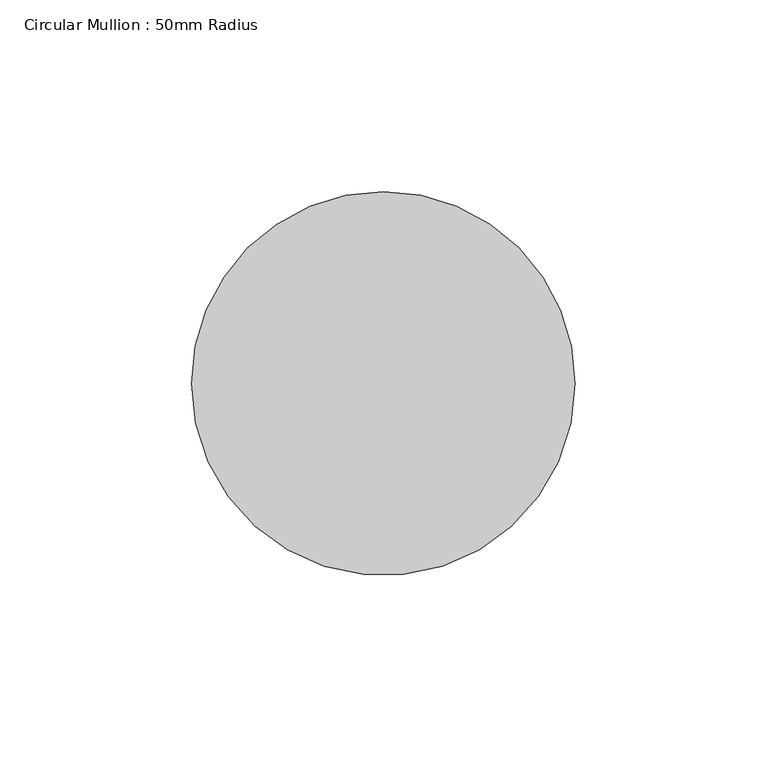
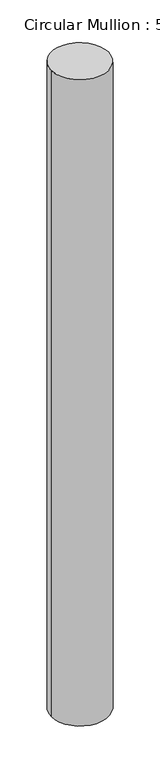
"""IFC4 building model written with IfcOpenShell, lengths in millimetres: member geometry, Circular Mullion : 50mm Radius."""

from ifc_helpers import new_model, si_unit, frame, origin, place, context, project, spatial, ellipse_curve, source, transform, mapped, element, save
from ifc_brep_helpers import plane_surface, cylinder_surface, advanced_brep


def circular_mullion_50mm_radius_43a44cb1(model_context):
    return source(origin(), model_context, "Body", "AdvancedBrep", [
        advanced_brep(
        [(-100.0, 0.0, 0.8091745), (0.0, 0.0, 0.0), (0.0, 0.0, -1191.2930542), (-100.0, 0.0, -1192.1357191)],
        [
            (0, 1, ellipse_curve(frame((-50.0, 0.0, 0.4045872), z_axis=(-0.00809072290162807, -0.013678510149129876, -0.9998737113070977), x_axis=(-0.5090365390349583, -0.8605981875941529, 0.015892181630306954)), 50.0063152, 50.0)),
            (1, 2),
            (2, 3, ellipse_curve(frame((-50.0, 0.0, -1191.7143867), z_axis=(-0.008425494316828716, -0.014244488524133757, 0.9998630434175488), x_axis=(0.5090311080034745, 0.8605890056681867, 0.016549755520753683)), 50.0068488, 50.0)),
            (3, 0),
            (1, 0, ellipse_curve(frame((-50.0, 0.0, 0.4045872), z_axis=(-0.00809072290162807, -0.013678510149129876, -0.9998737113070977), x_axis=(-0.5090365390349583, -0.8605981875941529, 0.015892181630306954)), 50.0063152, 50.0)),
            (3, 2, ellipse_curve(frame((-50.0, 0.0, -1191.7143867), z_axis=(-0.008425494316828716, -0.014244488524133757, 0.9998630434175488), x_axis=(0.5090311080034745, 0.8605890056681867, 0.016549755520753683)), 50.0068488, 50.0)),
        ],
        [
            cylinder_surface(frame((-50.0, 0.0, 0.0), z_axis=(0.0, 0.0, 1.0), x_axis=(1.0, 0.0, 0.0)), 50.0),
            plane_surface(frame((-262.3434586, 155.1739338, 0.0), z_axis=(0.00809072290162807, 0.013678510149129876, 0.9998737113070977), x_axis=(0.5090365390349586, 0.8605981875941526, -0.015892181630310483))),
            plane_surface(frame((-262.3434586, 155.1739338, -1191.2930542), z_axis=(0.008425494316828716, 0.014244488524133757, -0.9998630434175488), x_axis=(0.5090311080034744, 0.8605890056681866, 0.01654975552076499))),
        ],
        [
            (0, [[1, 2, 3, 4]]),
            (0, [[5, -4, 6, -2]]),
            (1, [[-1, -5]]),
            (2, [[-6, -3]]),
        ],
    ),
    ])


if __name__ == "__main__":
    model = new_model("IFC4")
    model_context = context("Model", 3, world=origin())
    ifc_project = project(units=[si_unit("LENGTHUNIT", "METRE", prefix="MILLI")], contexts=[model_context])
    site = spatial("IfcSite", under=ifc_project)
    building = spatial("IfcBuilding", under=site)
    placement = place(None, origin())
    circular_mullion_50mm_radius_shape = circular_mullion_50mm_radius_43a44cb1(model_context)
    element("IfcMember", 1, ObjectType="Circular Mullion : 50mm Radius", at=placement, inside=building, context=model_context, shape_type="MappedRepresentation", body=[
        mapped(circular_mullion_50mm_radius_shape, transform((0.0, 0.0, 0.0), x_axis=(1.0, 0.0, 0.0), y_axis=(0.0, 1.0, 0.0), z_axis=(0.0, 0.0, 1.0))),
    ])
    save(model, "model.ifc")

# Revit data of these elements
# Type "Circular Mullion : 50mm Radius"
#   built-in parameter 1007350 = 0.164042 (stored number, unit not read)
# Element 1 (IfcMember, "Circular Mullion : 50mm Radius")
#   Materials on its faces: "Aluminium"
# Materials
#   "Aluminium": class "Metal", colour RGB 247 247 247, transparency 0, Description = "Aluminium 6061", Cost = 0
